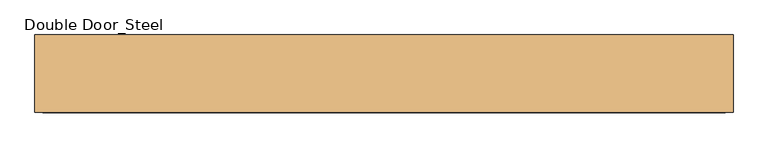
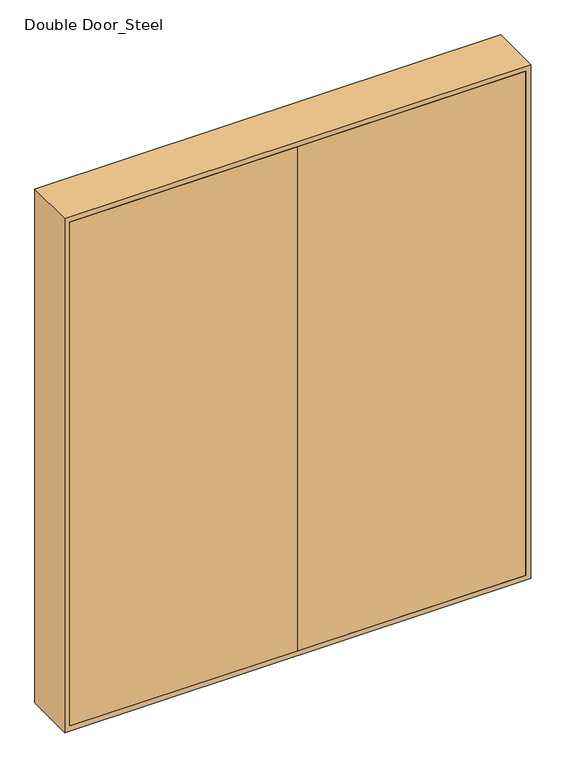
"""IFC4 building model written with IfcOpenShell, lengths in millimetres: door geometry, Double Door_Steel : H_DR_AR B12_Door_Double FSD 02."""

from ifc_helpers import new_model, si_unit, frame, origin, place, context, project, spatial, polyline, outline, extrude, faceted_brep, source, transform, mapped, element, save


def double_door_steel_63a69c0a(model_context):
    return source(origin(), model_context, "Body", "SolidModel", [
        extrude(outline(polyline([(880.0, -60.0), (880.0, -100.0), (0.0, -100.0), (0.0, -60.0), (880.0, -60.0)])), frame((0.0, 0.0, 20.0), z_axis=(0.0, 0.0, 1.0), x_axis=(1.0, 0.0, 0.0)), (0.0, 0.0, 1.0), 2060.0),
        extrude(outline(polyline([(0.0, -60.0), (0.0, -100.0), (-880.0, -100.0), (-880.0, -60.0), (0.0, -60.0)])), frame((0.0, 0.0, 20.0), z_axis=(0.0, 0.0, 1.0), x_axis=(1.0, 0.0, 0.0)), (0.0, 0.0, 1.0), 2060.0),
        faceted_brep([(900.0, 100.0, 2100.0), (-900.0, 100.0, 2100.0), (-900.0, -100.0, 2100.0), (900.0, -100.0, 2100.0), (865.0, -60.0, 2065.0), (-865.0, -60.0, 2065.0), (-865.0, 100.0, 2065.0), (865.0, 100.0, 2065.0), (880.0, -100.0, 2080.0), (-880.0, -100.0, 2080.0), (-880.0, -60.0, 2080.0), (880.0, -60.0, 2080.0), (-900.0, 100.0, 0.0), (-900.0, -100.0, 0.0), (-865.0, -60.0, 35.0), (-865.0, 100.0, 35.0), (-880.0, -100.0, 20.0), (-880.0, -60.0, 20.0), (900.0, -100.0, 0.0), (880.0, -100.0, 20.0), (900.0, 100.0, 0.0), (865.0, 100.0, 35.0), (865.0, -60.0, 35.0), (880.0, -60.0, 20.0)], [[[0, 1, 2, 3]], [[4, 5, 6, 7]], [[8, 9, 10, 11]], [[1, 12, 13, 2]], [[5, 14, 15, 6]], [[9, 16, 17, 10]], [[18, 3, 2, 13], [8, 19, 16, 9]], [[12, 20, 18, 13]], [[0, 20, 12, 1], [21, 7, 6, 15]], [[14, 22, 21, 15]], [[23, 11, 10, 17], [4, 22, 14, 5]], [[16, 19, 23, 17]], [[20, 0, 3, 18]], [[22, 4, 7, 21]], [[19, 8, 11, 23]]]),
    ])


if __name__ == "__main__":
    model = new_model("IFC4")
    model_context = context("Model", 3, world=origin())
    ifc_project = project(units=[si_unit("LENGTHUNIT", "METRE", prefix="MILLI")], contexts=[model_context])
    site = spatial("IfcSite", under=ifc_project)
    building = spatial("IfcBuilding", under=site)
    placement = place(None, origin())
    double_door_steel_shape = double_door_steel_63a69c0a(model_context)
    element("IfcDoor", 1, ObjectType="Double Door_Steel : H_DR_AR B12_Door_Double FSD 02", at=placement, inside=building, context=model_context, shape_type="MappedRepresentation", body=[
        mapped(double_door_steel_shape, transform((0.0, 0.0, 0.0), x_axis=(1.0, 0.0, 0.0), y_axis=(0.0, 1.0, 0.0), z_axis=(0.0, 0.0, 1.0))),
    ])
    save(model, "model.ifc")

# Revit data of these elements
# Type "Double Door_Steel : H_DR_AR B12_Door_Double FSD 02"
#   Type Mark = "FRD"
#   프레임 = ""
#   철물 = ""
#   유리/마감 = ""
#   위치/개소 = ""
#   부호 = "1/SD"
#   문번호 = ""
#   문기호 = "SD"
#   Analytic Construction = "<None>"
#   Height = 2100 mm
#   Width = 1800 mm
#   Define Thermal Properties by = 1
#   문 틀 = none
#   문 = none
#   Function = (empty or 0)
#   Assembly Code = ""
#   Wall Closure = (empty or 0)
